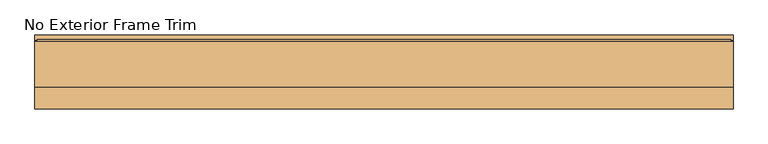
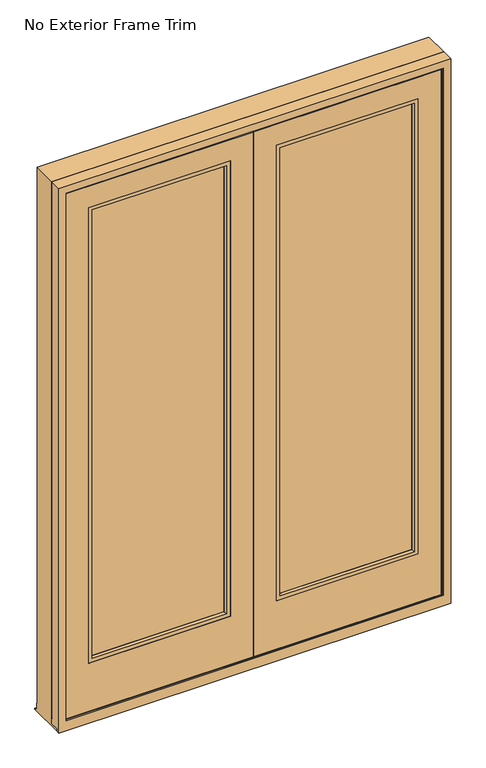
"""IFC4 building model written with IfcOpenShell, lengths in millimetres: door geometry, Door-In_Swing-Milgard-Essence-2_Panel : No Exterior Frame Trim."""

from ifc_helpers import new_model, si_unit, frame, origin, place, context, project, spatial, polyline, outline, extrude, faceted_brep, source, transform, mapped, element, save


def no_exterior_frame_trim_3783c24b(model_context):
    return source(origin(), model_context, "Body", "SolidModel", [
        extrude(outline(polyline([(591.4684989, -28.575), (591.4684989, -53.975), (54.2422052, -53.975), (54.2422052, -28.575), (591.4684989, -28.575)])), frame((0.0, 0.0, 245.0465023), z_axis=(0.0, 0.0, 1.0), x_axis=(1.0, 0.0, 0.0)), (0.0, 0.0, 1.0), 1856.965426),
        faceted_brep([(-22.501829, -56.3244996, 39.0524923), (-20.0336081, -53.2765006, 39.0524923), (47.7525111, -53.2765006, 39.0524923), (47.7525111, -55.0418002, 39.0524923), (61.9460004, -55.0418002, 39.0524923), (63.4695489, -53.975, 39.0524923), (66.9526032, -53.975, 39.0524923), (66.9526032, -55.857139, 39.0524923), (66.6827722, -56.3244996, 39.0524923), (579.0279319, -56.3244996, 39.0524923), (578.7581009, -55.857139, 39.0524923), (578.7581009, -53.975, 39.0524923), (582.2411552, -53.975, 39.0524923), (583.7647037, -55.0418002, 39.0524923), (597.9581931, -55.0418002, 39.0524923), (597.9581931, -53.2765006, 39.0524923), (665.7443122, -53.2765006, 39.0524923), (668.2125331, -56.3244996, 39.0524923), (685.524688, -56.3244996, 39.0524923), (685.524688, -64.6430002, 39.0524923), (-39.8139839, -64.6430002, 39.0524923), (-39.8139839, -56.3244996, 39.0524923), (-22.501829, -56.3244996, 56.3603664), (-20.0336081, -53.2765006, 58.8285873), (-22.501829, -56.3244996, 2178.7559624), (-20.0336081, -53.2765006, 2176.2877415), (-20.0336081, -53.2765006, 238.4932696), (-21.4631194, -55.0418002, 238.4932696), (-21.4631194, -55.0418002, 252.686759), (-20.5992417, -53.975, 254.2103075), (-20.5992417, -53.975, 257.6933617), (-22.1233678, -55.857139, 257.6933617), (-22.501829, -56.3244996, 257.4235308), (-39.8139839, -53.2765006, 58.8285873), (-39.8139839, -53.2765006, 238.4932696), (665.7443122, -53.2765006, 2176.2877415), (665.7443122, -53.2765006, 238.4932696), (685.524688, -53.2765006, 238.4932696), (685.524688, -53.2765006, 58.8285873), (665.7443122, -53.2765006, 58.8285873), (597.9581931, -53.2765006, 58.8285873), (47.7525111, -53.2765006, 58.8285873), (47.7525111, -53.2765006, 2108.5016224), (47.7525111, -53.2765006, 238.4932696), (597.9581931, -53.2765006, 238.4932696), (597.9581931, -53.2765006, 2108.5016224), (47.7525111, -55.0418002, 57.3990759), (47.7525111, -55.0418002, 2108.5016224), (47.7525111, -55.0418002, 257.6933617), (47.7525111, -53.975, 257.6933617), (47.7525111, -53.975, 254.2103075), (47.7525111, -55.0418002, 252.686759), (47.7525111, -55.0418002, 238.4932696), (61.9460004, -55.0418002, 57.3990759), (583.7647037, -55.0418002, 57.3990759), (597.9581931, -55.0418002, 57.3990759), (61.9460004, -55.0418002, 252.686759), (61.9460004, -55.0418002, 238.4932696), (597.9581931, -55.0418002, 2108.5016224), (597.9581931, -55.0418002, 257.6933617), (583.7647037, -55.0418002, 257.6933617), (583.7647037, -55.0418002, 2094.3081331), (61.9460004, -55.0418002, 2094.3081331), (61.9460004, -55.0418002, 257.6933617), (597.9581931, -55.0418002, 252.686759), (597.9581931, -55.0418002, 238.4932696), (583.7647037, -55.0418002, 238.4932696), (583.7647037, -55.0418002, 252.686759), (63.4695489, -53.975, 58.2629537), (63.4695489, -53.975, 254.2103075), (63.4695489, -53.975, 238.4932696), (63.4695489, -53.975, 2092.7845845), (63.4695489, -53.975, 257.6933617), (66.9526032, -53.975, 58.2629537), (578.7581009, -53.975, 58.2629537), (582.2411552, -53.975, 58.2629537), (582.2411552, -53.975, 2092.7845845), (582.2411552, -53.975, 257.6933617), (597.9581931, -53.975, 257.6933617), (597.9581931, -53.975, 254.2103075), (582.2411552, -53.975, 254.2103075), (582.2411552, -53.975, 238.4932696), (578.7581009, -53.975, 238.4932696), (578.7581009, -53.975, 254.2103075), (66.9526032, -53.975, 254.2103075), (66.9526032, -53.975, 238.4932696), (66.9526032, -53.975, 2089.3015303), (66.9526032, -53.975, 257.6933617), (578.7581009, -53.975, 257.6933617), (578.7581009, -53.975, 2089.3015303), (-39.8139839, -53.975, 254.2103075), (-39.8139839, -53.975, 257.6933617), (685.524688, -53.975, 257.6933617), (685.524688, -53.975, 254.2103075), (666.3099458, -53.975, 254.2103075), (666.3099458, -53.975, 257.6933617), (66.9526032, -55.857139, 56.7388275), (66.9526032, -55.0418002, 252.686759), (66.9526032, -55.0418002, 238.4932696), (66.9526032, -55.857139, 2089.3015303), (66.9526032, -55.857139, 257.6933617), (66.6827722, -56.3244996, 56.3603664), (62.3383529, -63.8492502, 2093.9157805), (62.3383529, -63.8492502, 253.0791115), (597.9581931, -63.8492502, 2108.5016224), (47.7525111, -63.8492502, 2108.5016224), (47.7525111, -63.8492502, 238.4932696), (597.9581931, -63.8492502, 238.4932696), (583.3723512, -63.8492502, 2093.9157805), (583.3723512, -63.8492502, 253.0791115), (47.7525111, -64.6430002, 2108.5016224), (47.7525111, -64.6430002, 238.4932696), (685.524688, -64.6430002, 2196.0681173), (-39.8139839, -64.6430002, 2196.0681173), (597.9581931, -64.6430002, 2108.5016224), (597.9581931, -64.6430002, 238.4932696), (-39.8139839, -56.3244996, 2196.0681173), (-39.8139839, -56.3244996, 257.4235308), (-39.8139839, -55.857139, 257.6933617), (-39.8139839, -55.0418002, 252.686759), (-39.8139839, -55.0418002, 238.4932696), (-39.8139839, -56.3244996, 56.3603664), (668.2125331, -56.3244996, 56.3603664), (685.524688, -56.3244996, 56.3603664), (685.524688, -56.3244996, 2196.0681173), (685.524688, -56.3244996, 257.4235308), (668.2125331, -56.3244996, 257.4235308), (668.2125331, -56.3244996, 2178.7559624), (578.7581009, -55.857139, 2089.3015303), (667.8340719, -55.857139, 257.6933617), (667.1738236, -55.0418002, 252.686759), (667.1738236, -55.0418002, 238.4932696), (578.7581009, -55.857139, 56.7388275), (578.7581009, -55.857139, 257.6933617), (578.7581009, -55.0418002, 238.4932696), (578.7581009, -55.0418002, 252.686759), (579.0279319, -56.3244996, 56.3603664), (685.524688, -55.0418002, 238.4932696), (685.524688, -55.0418002, 252.686759), (685.524688, -55.857139, 257.6933617)], [[[0, 1, 2, 3, 4, 5, 6, 7, 8, 9, 10, 11, 12, 13, 14, 15, 16, 17, 18, 19, 20, 21]], [[1, 0, 22, 23]], [[24, 25, 26, 27, 28, 29, 30, 31, 32]], [[2, 1, 23, 33, 34, 26, 25, 35, 36, 37, 38, 39, 16, 15, 40, 41], [42, 43, 44, 45]], [[3, 2, 41, 46]], [[42, 47, 48, 49, 50, 51, 52, 43]], [[4, 3, 46, 53]], [[14, 13, 54, 55]], [[52, 51, 56, 57]], [[47, 58, 59, 60, 61, 62, 63, 48]], [[64, 65, 66, 67]], [[5, 4, 53, 68]], [[57, 56, 69, 70]], [[62, 71, 72, 63]], [[6, 5, 68, 73]], [[12, 11, 74, 75]], [[71, 76, 77, 78, 79, 80, 81, 82, 83, 84, 85, 70, 69, 50, 49, 72], [86, 87, 88, 89]], [[90, 91, 30, 29]], [[92, 93, 94, 95]], [[7, 6, 73, 96]], [[85, 84, 97, 98]], [[86, 99, 100, 87]], [[8, 7, 96, 101]], [[99, 102, 103, 100]], [[104, 105, 106, 107], [102, 108, 109, 103]], [[106, 105, 110, 111]], [[20, 19, 112, 113], [114, 115, 111, 110]], [[21, 20, 113, 116, 117, 118, 91, 90, 119, 120, 34, 33, 121]], [[18, 17, 122, 123]], [[0, 21, 121, 22]], [[116, 124, 125, 126, 127, 24, 32, 117]], [[25, 24, 127, 35]], [[42, 45, 58, 47]], [[62, 61, 76, 71]], [[86, 89, 128, 99]], [[102, 99, 128, 108]], [[105, 104, 114, 110]], [[113, 112, 124, 116]], [[17, 16, 39, 122]], [[35, 127, 126, 129, 95, 94, 130, 131, 36]], [[15, 14, 55, 40]], [[58, 45, 44, 65, 64, 79, 78, 59]], [[13, 12, 75, 54]], [[81, 80, 67, 66]], [[76, 61, 60, 77]], [[11, 10, 132, 74]], [[128, 89, 88, 133]], [[83, 82, 134, 135]], [[10, 9, 136, 132]], [[108, 128, 133, 109]], [[114, 104, 107, 115]], [[124, 112, 19, 18, 123, 38, 37, 137, 138, 93, 92, 139, 125]], [[107, 106, 111, 115]], [[118, 117, 32, 31]], [[125, 139, 129, 126]], [[103, 109, 133, 100]], [[78, 77, 60, 59]], [[72, 49, 48, 63]], [[88, 87, 100, 133]], [[91, 118, 31, 30]], [[139, 92, 95, 129]], [[119, 90, 29, 28]], [[93, 138, 130, 94]], [[80, 79, 64, 67]], [[84, 83, 135, 97]], [[50, 69, 56, 51]], [[120, 119, 28, 27]], [[138, 137, 131, 130]], [[97, 135, 134, 98]], [[44, 43, 52, 57, 70, 85, 98, 134, 82, 81, 66, 65]], [[34, 120, 27, 26]], [[137, 37, 36, 131]], [[121, 33, 23, 22]], [[38, 123, 122, 39]], [[41, 40, 55, 54, 75, 74, 132, 136, 101, 96, 73, 68, 53, 46]], [[9, 8, 101, 136]]]),
        faceted_brep([(-39.8139839, -20.1929984, 39.0524923), (-39.8139839, -56.3244996, 39.0524923), (-39.8139839, -56.3244996, 2196.0681173), (-39.8139839, -20.1929984, 2196.0681173), (685.524688, -56.3244996, 39.0524923), (685.524688, -20.1929984, 39.0524923), (685.524688, -20.1929984, 2196.0681173), (685.524688, -56.3244996, 2196.0681173), (66.7863819, -27.3270033, 257.5271404), (578.9243222, -27.3270033, 257.5271404), (586.0583272, -20.1929984, 250.3931355), (59.6523769, -20.1929984, 250.3931355), (586.0583272, -20.1929984, 2096.6017565), (59.6523769, -20.1929984, 2096.6017565), (669.6356705, -56.3244996, 55.4786786), (-23.9249664, -56.3244996, 55.4786786), (-23.9249664, -56.3244996, 2180.1790999), (669.6356705, -56.3244996, 2180.1790999), (666.5876715, -53.2765006, 57.9468995), (-20.8769674, -53.2765006, 57.9468995), (666.5876715, -53.2765006, 2177.1311009), (-20.8769674, -53.2765006, 2177.1311009), (594.7531877, -53.2765006, 241.698275), (50.9575164, -53.2765006, 241.698275), (50.9575164, -53.2765006, 2105.296617), (594.7531877, -53.2765006, 2105.296617), (594.7531877, -50.8481081, 241.698275), (50.9575164, -50.8481081, 241.698275), (49.0643221, -50.8481081, 2107.1898114), (596.646382, -50.8481081, 2107.1898114), (596.646382, -50.8481081, 239.8050807), (49.0643221, -50.8481081, 239.8050807), (594.7531877, -50.8481081, 2105.296617), (50.9575164, -50.8481081, 2105.296617), (597.9581931, -46.8107689, 238.4932696), (47.7525111, -46.8107689, 238.4932696), (597.9581931, -27.8384005, 238.4932696), (581.6983611, -27.8384005, 238.4932696), (580.9617616, -28.575, 238.4932696), (578.9243222, -28.575, 238.4932696), (578.9243222, -27.8384005, 238.4932696), (66.7863819, -27.8384005, 238.4932696), (66.7863819, -28.575, 238.4932696), (64.7489425, -28.575, 238.4932696), (64.012343, -27.8384005, 238.4932696), (47.7525111, -27.8384005, 238.4932696), (597.9581931, -27.8384005, 254.7531016), (581.6983611, -27.8384005, 254.7531016), (578.9243222, -27.8384005, 254.7531016), (66.7863819, -27.8384005, 254.7531016), (64.012343, -27.8384005, 254.7531016), (47.7525111, -27.8384005, 254.7531016), (64.7489425, -28.575, 255.4897011), (47.7525111, -28.575, 255.4897011), (578.9243222, -28.575, 255.4897011), (66.7863819, -28.575, 255.4897011), (597.9581931, -28.575, 255.4897011), (580.9617616, -28.575, 255.4897011), (597.9581931, -28.575, 257.5271404), (580.9617616, -28.575, 257.5271404), (580.9617616, -28.575, 2091.505191), (64.7489425, -28.575, 2091.505191), (64.7489425, -28.575, 257.5271404), (47.7525111, -28.575, 257.5271404), (578.9243222, -28.575, 257.5271404), (66.7863819, -28.575, 257.5271404), (66.7863819, -28.575, 2089.4677516), (578.9243222, -28.575, 2089.4677516), (597.9581931, -27.8384005, 257.5271404), (581.6983611, -27.8384005, 257.5271404), (64.012343, -27.8384005, 257.5271404), (47.7525111, -27.8384005, 257.5271404), (66.7863819, -27.3270033, 2089.4677516), (64.012343, -27.8384005, 2092.2417904), (581.6983611, -27.8384005, 2092.2417904), (597.9581931, -27.8384005, 2108.5016224), (47.7525111, -27.8384005, 2108.5016224), (47.7525111, -46.8107689, 2108.5016224), (578.9243222, -27.3270033, 2089.4677516), (597.9581931, -46.8107689, 2108.5016224)], [[[0, 1, 2, 3]], [[4, 5, 6, 7]], [[8, 9, 10, 11]], [[0, 3, 6, 5], [11, 10, 12, 13]], [[4, 1, 0, 5]], [[2, 1, 4, 7], [14, 15, 16, 17]], [[15, 14, 18, 19]], [[20, 21, 19, 18], [22, 23, 24, 25]], [[23, 22, 26, 27]], [[28, 29, 30, 31], [27, 26, 32, 33]], [[31, 30, 34, 35]], [[35, 34, 36, 37, 38, 39, 40, 41, 42, 43, 44, 45]], [[37, 36, 46, 47]], [[41, 40, 48, 49]], [[45, 44, 50, 51]], [[51, 50, 52, 53]], [[49, 48, 54, 55]], [[47, 46, 56, 57]], [[53, 52, 43, 42, 55, 54, 39, 38, 57, 56, 58, 59, 60, 61, 62, 63], [64, 65, 66, 67]], [[9, 8, 65, 64]], [[59, 58, 68, 69]], [[63, 62, 70, 71]], [[13, 72, 8, 11]], [[55, 42, 41, 49]], [[72, 66, 65, 8]], [[43, 52, 50, 44]], [[61, 73, 70, 62]], [[73, 74, 69, 68, 75, 76, 71, 70]], [[76, 77, 35, 45, 51, 53, 63, 71]], [[77, 28, 31, 35]], [[33, 24, 23, 27]], [[19, 21, 16, 15]], [[13, 12, 78, 72]], [[66, 72, 78, 67]], [[61, 60, 74, 73]], [[76, 75, 79, 77]], [[28, 77, 79, 29]], [[33, 32, 25, 24]], [[21, 20, 17, 16]], [[6, 3, 2, 7]], [[78, 12, 10, 9]], [[39, 54, 48, 40]], [[67, 78, 9, 64]], [[74, 60, 59, 69]], [[57, 38, 37, 47]], [[79, 75, 68, 58, 56, 46, 36, 34]], [[30, 29, 79, 34]], [[25, 32, 26, 22]], [[17, 20, 18, 14]]]),
        extrude(outline(polyline([(-675.754549, -28.575), (-138.5282552, -28.575), (-138.5282552, -53.975), (-675.754549, -53.975), (-675.754549, -28.575)])), frame((0.0, 0.0, 245.0465023), z_axis=(0.0, 0.0, 1.0), x_axis=(1.0, 0.0, 0.0)), (0.0, 0.0, 1.0), 1856.965426),
        faceted_brep([(-61.784221, -56.3244996, 39.0524923), (-44.4720661, -56.3244996, 39.0524923), (-44.4720661, -64.6430002, 39.0524923), (-769.810738, -64.6430002, 39.0524923), (-769.810738, -56.3244996, 39.0524923), (-752.4985831, -56.3244996, 39.0524923), (-750.0303622, -53.2765006, 39.0524923), (-682.2442431, -53.2765006, 39.0524923), (-682.2442431, -55.0418002, 39.0524923), (-668.0507537, -55.0418002, 39.0524923), (-666.5272052, -53.975, 39.0524923), (-663.044151, -53.975, 39.0524923), (-663.044151, -55.857139, 39.0524923), (-663.3139819, -56.3244996, 39.0524923), (-150.9688223, -56.3244996, 39.0524923), (-151.2386532, -55.857139, 39.0524923), (-151.2386532, -53.975, 39.0524923), (-147.755599, -53.975, 39.0524923), (-146.2320504, -55.0418002, 39.0524923), (-132.0385611, -55.0418002, 39.0524923), (-132.0385611, -53.2765006, 39.0524923), (-64.252442, -53.2765006, 39.0524923), (-61.784221, -56.3244996, 2178.7559624), (-61.784221, -56.3244996, 257.4235308), (-62.1626822, -55.857139, 257.6933617), (-63.6868083, -53.975, 257.6933617), (-63.6868083, -53.975, 254.2103075), (-62.8229306, -55.0418002, 252.686759), (-62.8229306, -55.0418002, 238.4932696), (-64.252442, -53.2765006, 238.4932696), (-64.252442, -53.2765006, 2176.2877415), (-64.252442, -53.2765006, 58.8285873), (-61.784221, -56.3244996, 56.3603664), (-132.0385611, -53.2765006, 58.8285873), (-682.2442431, -53.2765006, 58.8285873), (-750.0303622, -53.2765006, 58.8285873), (-769.810738, -53.2765006, 58.8285873), (-769.810738, -53.2765006, 238.4932696), (-750.0303622, -53.2765006, 238.4932696), (-750.0303622, -53.2765006, 2176.2877415), (-44.4720661, -53.2765006, 238.4932696), (-44.4720661, -53.2765006, 58.8285873), (-132.0385611, -53.2765006, 2108.5016224), (-682.2442431, -53.2765006, 2108.5016224), (-682.2442431, -53.2765006, 238.4932696), (-132.0385611, -53.2765006, 238.4932696), (-132.0385611, -55.0418002, 238.4932696), (-132.0385611, -55.0418002, 252.686759), (-132.0385611, -53.975, 254.2103075), (-132.0385611, -53.975, 257.6933617), (-132.0385611, -55.0418002, 257.6933617), (-132.0385611, -55.0418002, 2108.5016224), (-132.0385611, -55.0418002, 57.3990759), (-146.2320504, -55.0418002, 257.6933617), (-146.2320504, -55.0418002, 2094.3081331), (-668.0507537, -55.0418002, 2094.3081331), (-668.0507537, -55.0418002, 257.6933617), (-682.2442431, -55.0418002, 257.6933617), (-682.2442431, -55.0418002, 2108.5016224), (-682.2442431, -55.0418002, 57.3990759), (-668.0507537, -55.0418002, 57.3990759), (-146.2320504, -55.0418002, 238.4932696), (-146.2320504, -55.0418002, 252.686759), (-682.2442431, -55.0418002, 252.686759), (-668.0507537, -55.0418002, 252.686759), (-668.0507537, -55.0418002, 238.4932696), (-682.2442431, -55.0418002, 238.4932696), (-146.2320504, -55.0418002, 57.3990759), (-147.755599, -53.975, 257.6933617), (-147.755599, -53.975, 2092.7845845), (-147.755599, -53.975, 238.4932696), (-147.755599, -53.975, 254.2103075), (-147.755599, -53.975, 58.2629537), (-151.2386532, -53.975, 238.4932696), (-151.2386532, -53.975, 254.2103075), (-663.044151, -53.975, 254.2103075), (-663.044151, -53.975, 238.4932696), (-666.5272052, -53.975, 238.4932696), (-666.5272052, -53.975, 254.2103075), (-682.2442431, -53.975, 254.2103075), (-682.2442431, -53.975, 257.6933617), (-666.5272052, -53.975, 257.6933617), (-666.5272052, -53.975, 2092.7845845), (-151.2386532, -53.975, 2089.3015303), (-663.044151, -53.975, 2089.3015303), (-663.044151, -53.975, 257.6933617), (-151.2386532, -53.975, 257.6933617), (-666.5272052, -53.975, 58.2629537), (-663.044151, -53.975, 58.2629537), (-769.810738, -53.975, 257.6933617), (-750.5959958, -53.975, 257.6933617), (-750.5959958, -53.975, 254.2103075), (-769.810738, -53.975, 254.2103075), (-151.2386532, -53.975, 58.2629537), (-44.4720661, -53.975, 254.2103075), (-44.4720661, -53.975, 257.6933617), (-151.2386532, -55.857139, 257.6933617), (-151.2386532, -55.857139, 2089.3015303), (-151.2386532, -55.0418002, 238.4932696), (-151.2386532, -55.0418002, 252.686759), (-151.2386532, -55.857139, 56.7388275), (-146.624403, -63.8492502, 253.0791115), (-146.624403, -63.8492502, 2093.9157805), (-150.9688223, -56.3244996, 56.3603664), (-682.2442431, -63.8492502, 2108.5016224), (-682.2442431, -63.8492502, 238.4932696), (-132.0385611, -63.8492502, 238.4932696), (-132.0385611, -63.8492502, 2108.5016224), (-667.6584012, -63.8492502, 253.0791115), (-667.6584012, -63.8492502, 2093.9157805), (-132.0385611, -64.6430002, 238.4932696), (-132.0385611, -64.6430002, 2108.5016224), (-44.4720661, -64.6430002, 2196.0681173), (-769.810738, -64.6430002, 2196.0681173), (-682.2442431, -64.6430002, 2108.5016224), (-682.2442431, -64.6430002, 238.4932696), (-44.4720661, -56.3244996, 56.3603664), (-44.4720661, -55.0418002, 238.4932696), (-44.4720661, -55.0418002, 252.686759), (-44.4720661, -55.857139, 257.6933617), (-44.4720661, -56.3244996, 257.4235308), (-44.4720661, -56.3244996, 2196.0681173), (-752.4985831, -56.3244996, 2178.7559624), (-752.4985831, -56.3244996, 257.4235308), (-769.810738, -56.3244996, 257.4235308), (-769.810738, -56.3244996, 2196.0681173), (-769.810738, -56.3244996, 56.3603664), (-752.4985831, -56.3244996, 56.3603664), (-663.044151, -55.857139, 2089.3015303), (-751.4598736, -55.0418002, 238.4932696), (-751.4598736, -55.0418002, 252.686759), (-752.120122, -55.857139, 257.6933617), (-663.044151, -55.857139, 56.7388275), (-663.044151, -55.0418002, 252.686759), (-663.044151, -55.0418002, 238.4932696), (-663.044151, -55.857139, 257.6933617), (-663.3139819, -56.3244996, 56.3603664), (-769.810738, -55.857139, 257.6933617), (-769.810738, -55.0418002, 252.686759), (-769.810738, -55.0418002, 238.4932696)], [[[0, 1, 2, 3, 4, 5, 6, 7, 8, 9, 10, 11, 12, 13, 14, 15, 16, 17, 18, 19, 20, 21]], [[22, 23, 24, 25, 26, 27, 28, 29, 30]], [[21, 31, 32, 0]], [[20, 33, 34, 7, 6, 35, 36, 37, 38, 39, 30, 29, 40, 41, 31, 21], [42, 43, 44, 45]], [[42, 45, 46, 47, 48, 49, 50, 51]], [[19, 52, 33, 20]], [[51, 50, 53, 54, 55, 56, 57, 58]], [[8, 59, 60, 9]], [[46, 61, 62, 47]], [[63, 64, 65, 66]], [[18, 67, 52, 19]], [[54, 53, 68, 69]], [[61, 70, 71, 62]], [[17, 72, 67, 18]], [[69, 68, 49, 48, 71, 70, 73, 74, 75, 76, 77, 78, 79, 80, 81, 82], [83, 84, 85, 86]], [[10, 87, 88, 11]], [[89, 90, 91, 92]], [[16, 93, 72, 17]], [[94, 26, 25, 95]], [[83, 86, 96, 97]], [[73, 98, 99, 74]], [[15, 100, 93, 16]], [[97, 96, 101, 102]], [[14, 103, 100, 15]], [[104, 105, 106, 107], [102, 101, 108, 109]], [[106, 110, 111, 107]], [[2, 112, 113, 3], [114, 111, 110, 115]], [[1, 116, 41, 40, 117, 118, 94, 95, 119, 120, 121, 112, 2]], [[0, 32, 116, 1]], [[121, 120, 23, 22, 122, 123, 124, 125]], [[4, 126, 127, 5]], [[30, 39, 122, 22]], [[42, 51, 58, 43]], [[54, 69, 82, 55]], [[83, 97, 128, 84]], [[102, 109, 128, 97]], [[107, 111, 114, 104]], [[112, 121, 125, 113]], [[39, 38, 129, 130, 91, 90, 131, 123, 122]], [[5, 127, 35, 6]], [[58, 57, 80, 79, 63, 66, 44, 43]], [[7, 34, 59, 8]], [[82, 81, 56, 55]], [[9, 60, 87, 10]], [[77, 65, 64, 78]], [[11, 88, 132, 12]], [[75, 133, 134, 76]], [[128, 135, 85, 84]], [[109, 108, 135, 128]], [[12, 132, 136, 13]], [[114, 115, 105, 104]], [[125, 124, 137, 89, 92, 138, 139, 37, 36, 126, 4, 3, 113]], [[105, 115, 110, 106]], [[101, 96, 135, 108]], [[124, 123, 131, 137]], [[119, 24, 23, 120]], [[68, 53, 50, 49]], [[95, 25, 24, 119]], [[80, 57, 56, 81]], [[85, 135, 96, 86]], [[137, 131, 90, 89]], [[48, 47, 62, 71]], [[74, 99, 133, 75]], [[78, 64, 63, 79]], [[92, 91, 130, 138]], [[118, 27, 26, 94]], [[99, 98, 134, 133]], [[138, 130, 129, 139]], [[117, 28, 27, 118]], [[40, 29, 28, 117]], [[44, 66, 65, 77, 76, 134, 98, 73, 70, 61, 46, 45]], [[139, 129, 38, 37]], [[33, 52, 67, 72, 93, 100, 103, 136, 132, 88, 87, 60, 59, 34]], [[116, 32, 31, 41]], [[36, 35, 127, 126]], [[13, 136, 103, 14]]]),
        faceted_brep([(-44.4720661, -20.1929984, 39.0524923), (-44.4720661, -20.1929984, 2196.0681173), (-44.4720661, -56.3244996, 2196.0681173), (-44.4720661, -56.3244996, 39.0524923), (-769.810738, -56.3244996, 39.0524923), (-769.810738, -56.3244996, 2196.0681173), (-769.810738, -20.1929984, 2196.0681173), (-769.810738, -20.1929984, 39.0524923), (-151.0724319, -27.3270033, 257.5271404), (-143.938427, -20.1929984, 250.3931355), (-670.3443772, -20.1929984, 250.3931355), (-663.2103723, -27.3270033, 257.5271404), (-143.938427, -20.1929984, 2096.6017565), (-670.3443772, -20.1929984, 2096.6017565), (-753.9217206, -56.3244996, 55.4786786), (-753.9217206, -56.3244996, 2180.1790999), (-60.3610836, -56.3244996, 2180.1790999), (-60.3610836, -56.3244996, 55.4786786), (-63.4090826, -53.2765006, 57.9468995), (-750.8737216, -53.2765006, 57.9468995), (-750.8737216, -53.2765006, 2177.1311009), (-63.4090826, -53.2765006, 2177.1311009), (-679.0392377, -53.2765006, 241.698275), (-679.0392377, -53.2765006, 2105.296617), (-135.2435664, -53.2765006, 2105.296617), (-135.2435664, -53.2765006, 241.698275), (-135.2435664, -50.8481081, 241.698275), (-679.0392377, -50.8481081, 241.698275), (-133.3503721, -50.8481081, 2107.1898114), (-133.3503721, -50.8481081, 239.8050807), (-680.9324321, -50.8481081, 239.8050807), (-680.9324321, -50.8481081, 2107.1898114), (-135.2435664, -50.8481081, 2105.296617), (-679.0392377, -50.8481081, 2105.296617), (-132.0385611, -46.8107689, 238.4932696), (-682.2442431, -46.8107689, 238.4932696), (-132.0385611, -27.8384005, 238.4932696), (-148.298393, -27.8384005, 238.4932696), (-149.0349925, -28.575, 238.4932696), (-151.0724319, -28.575, 238.4932696), (-151.0724319, -27.8384005, 238.4932696), (-663.2103723, -27.8384005, 238.4932696), (-663.2103723, -28.575, 238.4932696), (-665.2478116, -28.575, 238.4932696), (-665.9844111, -27.8384005, 238.4932696), (-682.2442431, -27.8384005, 238.4932696), (-132.0385611, -27.8384005, 254.7531016), (-148.298393, -27.8384005, 254.7531016), (-151.0724319, -27.8384005, 254.7531016), (-663.2103723, -27.8384005, 254.7531016), (-665.9844111, -27.8384005, 254.7531016), (-682.2442431, -27.8384005, 254.7531016), (-132.0385611, -28.575, 255.4897011), (-149.0349925, -28.575, 255.4897011), (-151.0724319, -28.575, 255.4897011), (-663.2103723, -28.575, 255.4897011), (-665.2478116, -28.575, 255.4897011), (-682.2442431, -28.575, 255.4897011), (-132.0385611, -28.575, 257.5271404), (-149.0349925, -28.575, 257.5271404), (-149.0349925, -28.575, 2091.505191), (-665.2478116, -28.575, 2091.505191), (-665.2478116, -28.575, 257.5271404), (-682.2442431, -28.575, 257.5271404), (-663.2103723, -28.575, 257.5271404), (-663.2103723, -28.575, 2089.4677516), (-151.0724319, -28.575, 2089.4677516), (-151.0724319, -28.575, 257.5271404), (-132.0385611, -27.8384005, 257.5271404), (-148.298393, -27.8384005, 257.5271404), (-665.9844111, -27.8384005, 257.5271404), (-682.2442431, -27.8384005, 257.5271404), (-151.0724319, -27.3270033, 2089.4677516), (-148.298393, -27.8384005, 2092.2417904), (-132.0385611, -27.8384005, 2108.5016224), (-682.2442431, -27.8384005, 2108.5016224), (-665.9844111, -27.8384005, 2092.2417904), (-132.0385611, -46.8107689, 2108.5016224), (-663.2103723, -27.3270033, 2089.4677516), (-682.2442431, -46.8107689, 2108.5016224)], [[[0, 1, 2, 3]], [[4, 5, 6, 7]], [[8, 9, 10, 11]], [[0, 7, 6, 1], [9, 12, 13, 10]], [[4, 7, 0, 3]], [[2, 5, 4, 3], [14, 15, 16, 17]], [[17, 18, 19, 14]], [[20, 19, 18, 21], [22, 23, 24, 25]], [[25, 26, 27, 22]], [[28, 29, 30, 31], [26, 32, 33, 27]], [[29, 34, 35, 30]], [[34, 36, 37, 38, 39, 40, 41, 42, 43, 44, 45, 35]], [[36, 46, 47, 37]], [[40, 48, 49, 41]], [[44, 50, 51, 45]], [[46, 52, 53, 47]], [[48, 54, 55, 49]], [[50, 56, 57, 51]], [[52, 58, 59, 60, 61, 62, 63, 57, 56, 43, 42, 55, 54, 39, 38, 53], [64, 65, 66, 67]], [[11, 64, 67, 8]], [[58, 68, 69, 59]], [[62, 70, 71, 63]], [[12, 9, 8, 72]], [[54, 48, 40, 39]], [[72, 8, 67, 66]], [[38, 37, 47, 53]], [[60, 59, 69, 73]], [[73, 69, 68, 74, 75, 71, 70, 76]], [[74, 68, 58, 52, 46, 36, 34, 77]], [[77, 34, 29, 28]], [[32, 26, 25, 24]], [[18, 17, 16, 21]], [[12, 72, 78, 13]], [[66, 65, 78, 72]], [[60, 73, 76, 61]], [[74, 77, 79, 75]], [[28, 31, 79, 77]], [[32, 24, 23, 33]], [[21, 16, 15, 20]], [[6, 5, 2, 1]], [[78, 11, 10, 13]], [[42, 41, 49, 55]], [[65, 64, 11, 78]], [[56, 50, 44, 43]], [[76, 70, 62, 61]], [[79, 35, 45, 51, 57, 63, 71, 75]], [[30, 35, 79, 31]], [[23, 22, 27, 33]], [[15, 14, 19, 20]]]),
        faceted_brep([(719.8791802, -74.6125, 0.0), (719.8791802, -61.9125011, 0.0), (719.8791802, -61.9125011, 9.128125), (719.8791802, -27.7018482, 9.128125), (719.8791802, -27.6987011, 2235.2), (719.8791802, -74.6125, 2235.2), (-804.1208198, -61.9125011, 0.0), (-804.1208198, -74.6125, 0.0), (-804.1208198, -74.6125, 2235.2), (-804.1208198, -27.6987011, 2235.2), (-804.1208198, -27.7018482, 9.128125), (-804.1208198, -61.9125011, 9.128125), (-775.5465905, -74.6125, 41.6602461), (-775.5465905, -74.6125, 2206.6257706), (691.3049508, -74.6125, 2206.6257706), (691.3049508, -74.6125, 41.6602461), (-773.0058163, -61.9125011, 9.128125), (-773.0058163, -61.9125011, 40.5405728), (688.7641767, -61.9125011, 40.5405728), (688.7641767, -61.9125011, 9.128125), (693.7179256, -27.7018482, 9.128125), (688.7641767, -55.02769, 9.128125), (691.304169, -55.02769, 9.128125), (691.304169, -50.2285006, 9.128125), (693.7179256, -50.2285006, 9.128125), (-777.9595653, -27.7018482, 9.128125), (-777.9595653, -50.2285006, 9.128125), (-775.5458087, -50.2285006, 9.128125), (-775.5458087, -55.02769, 9.128125), (-773.0058163, -55.02769, 9.128125), (-773.0058163, -66.2127992, 41.2988289), (-775.5465905, -66.2127992, 41.2988289), (-775.5465905, -68.2625043, 41.6602461), (691.3049508, -68.2625043, 41.6602461), (691.3049508, -66.2127992, 41.2988289), (688.7641767, -66.2127992, 41.2988289), (691.3049508, -66.2127992, 2206.6257706), (-775.5465905, -66.2127992, 2206.6257706), (-773.0058163, -66.2127992, 2204.0849965), (688.7641767, -66.2127992, 2204.0849965), (-773.0058163, -55.02769, 2204.0849965), (688.7641767, -55.02769, 2204.0849965), (-775.5458087, -55.02769, 2206.6249888), (691.304169, -55.02769, 2206.6249888), (-777.9595653, -27.6987011, 2209.0380233), (693.7179256, -27.6987011, 2209.0380233), (693.7179256, -50.2285006, 2209.0380233), (-777.9595653, -50.2285006, 2209.0380233), (691.304169, -50.2285006, 2206.6249888), (-775.5458087, -50.2285006, 2206.6249888)], [[[0, 1, 2, 3, 4, 5]], [[6, 7, 8, 9, 10, 11]], [[8, 7, 0, 5], [12, 13, 14, 15]], [[1, 6, 11, 16, 17, 18, 19, 2]], [[1, 0, 7, 6]], [[20, 3, 2, 19, 21, 22, 23, 24]], [[25, 26, 27, 28, 29, 16, 11, 10]], [[18, 17, 30, 31, 32, 33, 34, 35]], [[12, 15, 33, 32]], [[36, 37, 31, 30, 38, 39, 35, 34]], [[39, 38, 40, 41]], [[41, 40, 29, 28, 42, 43, 22, 21]], [[44, 45, 46, 47]], [[4, 3, 20, 45, 44, 25, 10, 9]], [[5, 4, 9, 8]], [[37, 36, 14, 13]], [[15, 14, 36, 34, 33]], [[41, 21, 19, 18, 35, 39]], [[23, 22, 43, 48]], [[24, 23, 48, 49, 27, 26, 47, 46]], [[20, 24, 46, 45]], [[48, 43, 42, 49]], [[13, 12, 32, 31, 37]], [[29, 40, 38, 30, 17, 16]], [[42, 28, 27, 49]], [[26, 25, 44, 47]]]),
        faceted_brep([(719.8791802, 87.2170398, 0.0007738), (719.8791802, 87.2170398, 3.8703788), (719.8791802, 74.5870975, 4.9752253), (719.8791802, 74.5870975, 32.7181022), (719.8791802, 72.3899958, 33.0268847), (719.8791802, 72.3899958, 2235.2), (719.8791802, -27.7018482, 2235.2), (719.8791802, -27.7018482, 34.0993068), (719.8791802, -55.5625016, 36.0475021), (719.8791802, -55.5625016, 39.2302591), (719.8791802, -61.9125011, 40.9473783), (719.8791802, -61.9125011, 0.0007738), (-804.1208198, -61.9125011, 0.0007738), (-804.1208198, -61.9125011, 40.9473783), (-804.1208198, -55.5625016, 39.2302591), (-804.1208198, -55.5625016, 36.0475021), (-804.1208198, -27.7018482, 34.0993068), (-804.1208198, -27.7018482, 2235.2), (-804.1208198, 72.3899958, 2235.2), (-804.1208198, 72.3899958, 33.0268847), (-804.1208198, 74.5870975, 32.7181022), (-804.1208198, 74.5870975, 4.9752253), (-804.1208198, 87.2170398, 3.8703788), (-804.1208198, 87.2170398, 0.0007738), (-799.2955843, 74.5870975, 4.9752253), (-799.2955843, 76.1999992, 4.8341313), (-775.5465905, 76.1999992, 4.8341313), (-775.5465905, 74.5870975, 4.9752253), (691.3049508, 74.5870975, 4.9752253), (691.3049508, 76.1999992, 4.8341313), (715.0539447, 76.1999992, 4.8341313), (715.0539447, 74.5870975, 4.9752253), (715.0539447, 74.5870975, 32.7181022), (-799.2955843, 74.5870975, 32.7181022), (-775.5465905, 74.5870975, 32.7181022), (691.3049508, 74.5870975, 32.7181022), (715.0539447, 68.8467009, 33.5248623), (717.7209545, 68.8467009, 33.5248623), (717.7209545, 72.3899958, 33.0268847), (-801.9625942, 72.3899958, 33.0268847), (-801.9625942, 68.8467009, 33.5248623), (-799.2955843, 68.8467009, 33.5248623), (-775.5465905, 68.8467009, 33.5248623), (691.3049508, 68.8467009, 33.5248623), (-775.5465905, 68.8467009, 17.4625), (691.3049508, 68.8467009, 17.4625), (715.0539447, 68.8467009, 17.4625), (717.7209545, 68.8467009, 17.4625), (-801.9625942, 68.8467009, 17.4625), (-799.2955843, 68.8467009, 17.4625), (-775.5465905, 53.8860989, 17.4625), (691.3049508, 53.8860989, 17.4625), (715.0539447, 65.2779957, 17.4625), (717.7209545, 65.2779957, 17.4625), (-801.9625942, 65.2779957, 17.4625), (-799.2955843, 65.2779957, 17.4625), (-775.5465905, 53.8860989, 34.8617092), (691.3049508, 53.8860989, 34.8617092), (-775.5465905, 53.3399975, 34.9482004), (-764.4279497, 53.3399975, 34.9482004), (-761.2119699, 7.3532983, 42.2315423), (676.9703302, 7.3532983, 42.2315423), (680.1863101, 53.3399975, 34.9482004), (691.3049508, 53.3399975, 34.9482004), (-761.2119699, 7.3532983, 53.8407291), (676.9703302, 7.3532983, 53.8407291), (-759.6577128, -14.8717015, 57.7596273), (675.4160732, -14.8717015, 57.7596273), (678.8330892, -14.8717015, 57.7596273), (681.6271165, -14.8717015, 57.7596273), (681.6271165, -7.5583358, 56.4700734), (678.8330892, -7.5583358, 56.4700734), (-765.8687562, -14.8717015, 57.7596273), (-763.0747288, -14.8717015, 57.7596273), (-763.0747288, -7.5583358, 56.4700734), (-765.8687562, -7.5583358, 56.4700734), (-759.6577128, -14.8717015, 33.2021408), (675.4160732, -14.8717015, 33.2021408), (678.8330892, -14.8717015, 33.2021408), (681.6271165, -14.8717015, 33.2021408), (-765.8687562, -14.8717015, 33.2021408), (-763.0747288, -14.8717015, 33.2021408), (693.7179256, -27.7018482, 34.0993068), (693.7179256, -50.295149, 35.6791751), (691.3049508, -50.295149, 35.6791751), (691.3049508, -15.6806239, 33.2587058), (681.6271165, -15.6806239, 33.2587058), (678.8330892, -15.6806239, 33.2587058), (675.3595029, -15.6806239, 33.2587058), (-759.6011426, -15.6806239, 33.2587058), (-763.0747288, -15.6806239, 33.2587058), (-765.8687562, -15.6806239, 33.2587058), (-775.5465905, -15.6806239, 33.2587058), (-775.5465905, -50.295149, 35.6791751), (-777.9595653, -50.295149, 35.6791751), (-777.9595653, -27.7018482, 34.0993068), (691.3049508, 53.3399975, 2206.6257706), (691.3049508, 76.1999992, 2206.6257706), (-775.5465905, 76.1999992, 2206.6257706), (-799.2955843, 76.1999992, 2230.3747645), (715.0539447, 76.1999992, 2230.3747645), (715.0539447, 65.2779957, 2230.3747645), (-799.2955843, 65.2779957, 2230.3747645), (-801.9625942, 65.2779957, 2233.0417743), (717.7209545, 65.2779957, 2233.0417743), (717.7209545, 72.3899958, 2233.0417743), (-801.9625942, 72.3899958, 2233.0417743), (-777.9595653, -27.7018482, 2209.0387455), (693.7179256, -27.7018482, 2209.0387455), (693.7179256, -50.295149, 2209.0387455), (-777.9595653, -50.295149, 2209.0387455), (-775.5465905, -50.295149, 2206.6257706), (691.3049508, -50.295149, 2206.6257706), (691.3049508, -15.6806239, 2206.6257706), (-775.5465905, -15.6806239, 2206.6257706), (-765.8687562, -15.6806239, 2196.9479363), (681.6271165, -15.6806239, 2196.9479363), (681.6271165, -7.5583358, 2196.9479363), (-765.8687562, -7.5583358, 2196.9479363), (-763.0747288, -7.5583358, 2194.153909), (678.8330892, -7.5583358, 2194.153909), (678.8330892, -15.6806239, 2194.153909), (-763.0747288, -15.6806239, 2194.153909), (-759.6011426, -15.6806239, 2190.6803228), (675.3595029, -15.6806239, 2190.6803228), (680.1863101, 53.3399975, 2195.5071299), (-764.4279497, 53.3399975, 2195.5071299), (-775.5465905, 53.3399975, 2206.6257706)], [[[0, 1, 2, 3, 4, 5, 6, 7, 8, 9, 10, 11]], [[12, 13, 14, 15, 16, 17, 18, 19, 20, 21, 22, 23]], [[1, 0, 23, 22]], [[2, 1, 22, 21, 24, 25, 26, 27, 28, 29, 30, 31]], [[3, 2, 31, 32]], [[21, 20, 33, 24]], [[28, 27, 34, 35]], [[4, 3, 32, 36, 37, 38]], [[20, 19, 39, 40, 41, 33]], [[35, 34, 42, 43]], [[43, 42, 44, 45]], [[37, 36, 46, 47]], [[41, 40, 48, 49]], [[45, 44, 50, 51]], [[47, 46, 52, 53]], [[49, 48, 54, 55]], [[51, 50, 56, 57]], [[57, 56, 58, 59, 60, 61, 62, 63]], [[61, 60, 64, 65]], [[65, 64, 66, 67]], [[68, 69, 70, 71]], [[72, 73, 74, 75]], [[67, 66, 76, 77]], [[69, 68, 78, 79]], [[73, 72, 80, 81]], [[15, 8, 7, 82, 83, 84, 85, 86, 79, 78, 87, 88, 77, 76, 89, 90, 81, 80, 91, 92, 93, 94, 95, 16]], [[9, 8, 15, 14]], [[10, 9, 14, 13]], [[11, 10, 13, 12]], [[12, 23, 0, 11]], [[96, 97, 29, 28, 35, 43, 45, 51, 57, 63]], [[97, 98, 26, 25, 99, 100, 30, 29]], [[100, 101, 52, 46, 36, 32, 31, 30]], [[101, 102, 55, 54, 103, 104, 53, 52]], [[104, 105, 38, 37, 47, 53]], [[105, 106, 39, 19, 18, 5, 4, 38]], [[6, 17, 16, 95, 107, 108, 82, 7]], [[108, 109, 83, 82]], [[109, 110, 94, 93, 111, 112, 84, 83]], [[112, 113, 85, 84]], [[113, 114, 92, 91, 115, 116, 86, 85]], [[116, 117, 70, 69, 79, 86]], [[117, 118, 75, 74, 119, 120, 71, 70]], [[120, 121, 87, 78, 68, 71]], [[121, 122, 90, 89, 123, 124, 88, 87]], [[124, 125, 62, 61, 65, 67, 77, 88]], [[125, 126, 59, 58, 127, 96, 63, 62]], [[97, 96, 127, 98]], [[100, 99, 102, 101]], [[104, 103, 106, 105]], [[5, 18, 17, 6]], [[108, 107, 110, 109]], [[112, 111, 114, 113]], [[116, 115, 118, 117]], [[120, 119, 122, 121]], [[124, 123, 126, 125]], [[98, 127, 58, 56, 50, 44, 42, 34, 27, 26]], [[102, 99, 25, 24, 33, 41, 49, 55]], [[106, 103, 54, 48, 40, 39]], [[110, 107, 95, 94]], [[114, 111, 93, 92]], [[118, 115, 91, 80, 72, 75]], [[122, 119, 74, 73, 81, 90]], [[126, 123, 89, 76, 66, 64, 60, 59]]]),
    ])


if __name__ == "__main__":
    model = new_model("IFC4")
    model_context = context("Model", 3, world=origin())
    ifc_project = project(units=[si_unit("LENGTHUNIT", "METRE", prefix="MILLI")], contexts=[model_context])
    site = spatial("IfcSite", under=ifc_project)
    building = spatial("IfcBuilding", under=site)
    placement = place(None, origin())
    no_exterior_frame_trim_shape = no_exterior_frame_trim_3783c24b(model_context)
    element("IfcDoor", 1, ObjectType="Door-In_Swing-Milgard-Essence-2_Panel : No Exterior Frame Trim", at=placement, inside=building, context=model_context, shape_type="MappedRepresentation", body=[
        mapped(no_exterior_frame_trim_shape, transform((0.0, 0.0, 0.0), x_axis=(1.0, 0.0, 0.0), y_axis=(0.0, 1.0, 0.0), z_axis=(0.0, 0.0, 1.0))),
    ])
    save(model, "model.ifc")

# Revit data of these elements
# Type "Door-In_Swing-Milgard-Essence-2_Panel : No Exterior Frame Trim"
#   Type Mark = "25"
#   Version = "2014 - v1.0a"
#   STC Ratings = ""
#   Product data url = "https://bimobject.com/milgardwindowsanddoors/product/milgard-310"
#   Performance Ratings = "https://www.milgard.com/sites/default/files/new-series/essence-series/essence-series-french-style-sliding-doors/field_series_detail_ratings_file/efsd_performance_chart.pdf"
#   Max/Min Note [instance default] = "MIN (5' x 6' 8'') / MAX (6' x 8')"
#   Installation Service and URL = "https://www.milgard.com/professionals/installation-finishing"
#   Frame Type = "4 9/16'' Wall Condition"
#   Exterior Trim = "Not Available"
#   Copyright = "Copyright © 2017 Milgard Manufacturing Inc. All Rights Reserved."
#   Warranty URL = "https://www.milgard.com/learn/understanding-your-full-lifetime-warranty"
#   Video Link = "https://www.youtube.com/user/MilgardWindows"
#   URL = "https://www.milgard.com"
#   Product Documentation Link = "https://www.milgard.com/professionals/essence-series-patio-doors/essence-series-swing-french-doors-new#series-styles--wrapper"
#   Performance URL = "https://www.milgard.com/sites/default/files/series-detail/files/ratings/essence_is-os_performance_ratings_0.pdf"
#   Material = ""
#   Size Note = "Essence Series doors are custom built to size and specifications"
#   Manufacturer Phone Number = "1-800-Milgard"
#   Manufacturer Address = "1010 54th Avenue East, Tacoma, WA 98424"
#   Keynote = "08 14 00"
#   Product Page URL = "https://www.milgard.com/professionals/essence-series-patio-doors/essence-series-swing-french-doors-new#series-styles--wrapper"
#   Product Name = "Essence Series In-Swing French Door, 2 Panel"
#   Operation = "In-Swing"
#   Model = "Essence"
#   Manufacturer = "Milgard Window & Doors"
#   Inset Note [instance default] = "To set Door into wall use Inset parameter found in Instance Properties."
#   Grid Style [instance default] = "Select ‘Grid Style’"
#   Grid Pattern [instance default] = "Select ‘Grid Pattern'"
#   Description = "In-Swing Door, 2 Panel"
#   Construction Type = "-"
#   Assembly Code = "B2030"
#   Analytic Construction = "<None>"
#   Vent Opening Width [instance default] = 2' - 0.05664"
#   Vent Opening Height [instance default] = 7' - 0"
#   Vent Opening Area - Overall [instance default] = 28.0661 SF
#   Vent Opening Area - Individual [instance default] = 14.033 SF
#   Frame Width [instance default] = 5' - 0"
#   Frame Height [instance default] = 7' - 4"
#   Door Swing [instance default] = 90.00°
#   Daylight Opening Width [instance default] = 1' - 8 3/16"
#   Daylight Opening Height [instance default] = 5' - 11 7/8"
#   Daylight Opening Area - Overall [instance default] = 20.1525 SF
#   Daylight Opening Area - Individual [instance default] = 10.0762 SF
#   Width C Min [instance default] = 5' - 0"
#   Wall Width [instance default] = 1' - 0"
#   Individual Door Panel Width [instance default] = 2' - 4.55664"
#   Individual Door Panel Height [instance default] = 7' - 0 59/64"
#   Jamb Extension [instance default] = 0' - 6 1/16"
#   Height C Min [instance default] = 7' - 4"
#   Thermal Resistance (R) = 1.7611 (m²·K)/W
#   Side to Glazing = 0' - 5 5/128"
#   Rough Width [instance default] = 5' - 1"
#   Rough Offset = 0' - 0 1/2"
#   Rough Height [instance default] = 7' - 4 1/2"
#   Inset Offset [instance default] = 0' - 0"
#   Inset [instance default] = 0' - 0"
#   Height [instance default] = 7' - 4"
#   Heat Transfer Coefficient (U) = 0.567826 W/(m²·K)
#   Glazing Thickness = 0' - 1"
#   Glass Width [instance default] = 1' - 9.11914"
#   Glass Height [instance default] = 6' - 0 13/16"
#   Top to Glazing = 0' - 5 1/8"
#   Width [instance default] = 6' - 0"
#   Call Out Width [instance default] = 5' - 0"
#   Call Out Height [instance default] = 7' - 4"
#   Center to Interior = 0' - 1 5/16"
#   Center to Exterior = 0' - 4 5/8"
#   C Panel Height [instance default] = 7' - 0 59/64"
#   C Panel Width [instance default] = 2' - 4.55664"
#   C Door Swing [instance default] = 90.00°
#   C Brick Mold = 0' - 0"
#   Bottom to Glazing = 0' - 10 1/256"
#   Warning Text [instance default] = yes
#   Overall Min Max [instance default] = no
#   Operation Symbol [instance default] = yes
#   Min Max Text [instance default] = no
#   Grid Visibility C [instance default] = no
#   Ext Flat = no
#   Ext Brickmould = no
#   Jamb Extension by Others [instance default] = no
#   Interior Trim by Others [instance default] = no
#   Grid Style - Simulated Divide Lite (3/4in) [instance default] = no
#   Grid Style - Simulated Divide Lite (2-1/4in) [instance default] = no
#   Grid Style - Simulated Divide Lite (1-1/8in) [instance default] = no
#   Grid Style - Grids Between Glass (5/8in) [instance default] = no
#   Grid Style - Grids Between Glass (1-1/16in) [instance default] = no
#   Grid Pattern - Standard [instance default] = no
#   Flat Trim = no
#   Ext Trim Visible = no
#   Constraint = 1
#   C Jamb Extension Visibility [instance default] = no
#   Brick Mold = no
#   Interior Frame = Wood - Milgard - Douglas Fir
#   Glazing Material = Glass - Milgard - SunCoat Low-E2
#   Exterior Frame = Fiberglass - Milgard - Powder Coat, Frost
#   Visual Light Transmittance = 0
#   Solar Heat Gain Coefficient = 0
#   Wall Closure = (empty or 0)
# Element 1 (IfcDoor, "Door-In_Swing-Milgard-Essence-2_Panel : No Exterior Frame Trim")
#   Wall Width = 0' - 6"
#   Jamb Extension = 0' - 0 1/16"
#   Materials on its faces: "Fiberglass - Milgard - Powder Coat, Frost", "Wood - Milgard - Douglas Fir", "Glass - Milgard - SunCoat Low-E2"
# Materials
#   "Wood - Milgard - Douglas Fir": class "Wood", colour RGB 204 153 0, transparency 0, Keynote = "06 01 00", Model = "Douglas Fir", Manufacturer = "Milgard", URL = "https://www.milgard.com", Description = "Clear Vertical Grain Douglas Fir", Cost = 0
#   "Glass - Milgard - SunCoat Low-E2": class "Glass", colour RGB 218 227 224, transparency 0.7, Keynote = "08 81 00.A1", Model = "Suncoat", Manufacturer = "Milgard", URL = "https://www.milgard.com", Description = "SunCoat Low-E2 Glass", Cost = 0
#   "Fiberglass - Milgard - Powder Coat, Frost": class "Fiberglass", colour RGB 236 242 252, transparency 0, Keynote = "09 91 00.A1", Model = "Frost", Manufacturer = "Milgard", URL = "https://www.milgard.com", Description = "Powder Coat, Frost", Cost = 0
